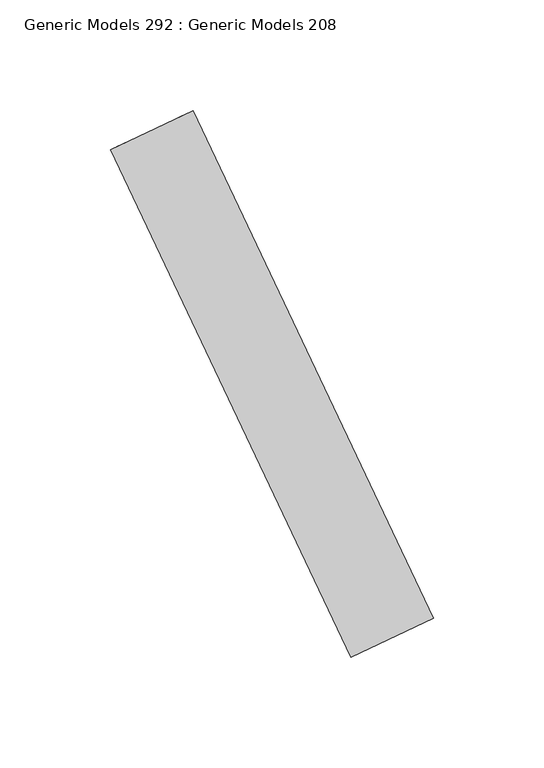
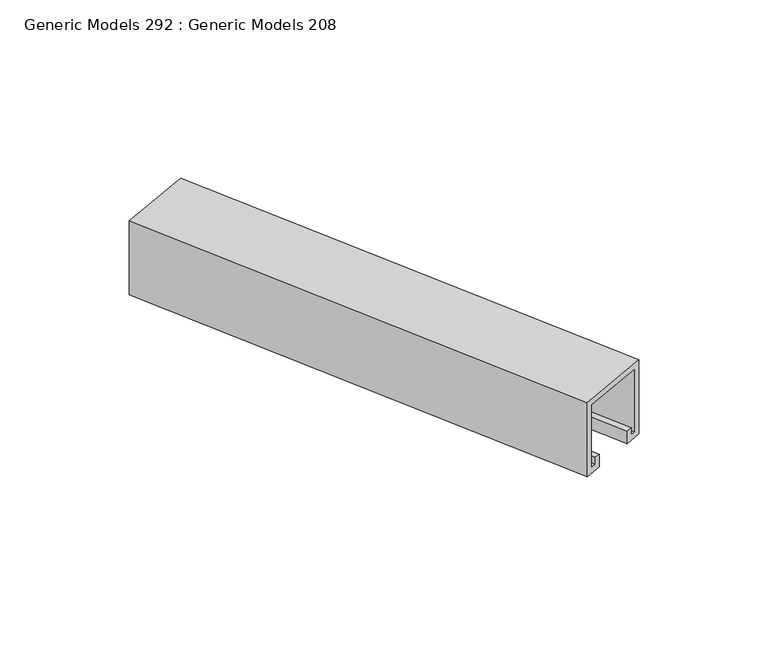
"""IFC4 building model written with IfcOpenShell, lengths in millimetres: proxy geometry, Generic Models 292 : Generic Models 208."""

from ifc_helpers import new_model, si_unit, frame, origin, place, context, project, spatial, polyline, outline, extrude, source, transform, mapped, element, save


def generic_models_292_generic_models_208_bf7aaf75(model_context):
    return source(origin(), model_context, "Body", "SweptSolid", [
        extrude(outline(polyline([(-3.175, 0.0), (-3.175, 34.925), (-38.1, 34.925), (-38.1, 31.75), (-34.13125, 31.75), (-34.13125, 28.575), (-41.275, 28.575), (-41.275, 38.1), (0.0, 38.1), (0.0, -3.175), (-41.275, -3.175), (-41.275, 6.35), (-34.13125, 6.35), (-34.13125, 3.175), (-38.1, 3.175), (-38.1, 0.0), (-3.175, 0.0)])), frame((-2064.1591152, -22579.8272705, 1035.05), z_axis=(-0.4281549299436163, 0.9037053479785195, 0.0), x_axis=(0.0, 0.0, 1.0)), (0.0, 0.0, 1.0), 254.0),
    ])


if __name__ == "__main__":
    model = new_model("IFC4")
    model_context = context("Model", 3, world=origin())
    ifc_project = project(units=[si_unit("LENGTHUNIT", "METRE", prefix="MILLI")], contexts=[model_context])
    site = spatial("IfcSite", under=ifc_project)
    building = spatial("IfcBuilding", under=site)
    placement = place(None, origin())
    generic_models_292_generic_models_208_shape = generic_models_292_generic_models_208_bf7aaf75(model_context)
    element("IfcBuildingElementProxy", 1, Name="Generic Models 292 : Generic Models 208", ObjectType="Generic Models 292 : Generic Models 208", at=placement, inside=building, context=model_context, shape_type="MappedRepresentation", body=[
        mapped(generic_models_292_generic_models_208_shape, transform((0.0, 0.0, 0.0), x_axis=(1.0, 0.0, 0.0), y_axis=(0.0, 1.0, 0.0), z_axis=(0.0, 0.0, 1.0))),
    ])
    save(model, "model.ifc")

# Revit data of these elements
# Element 1 (IfcBuildingElementProxy, "Generic Models 292 : Generic Models 208")
#   Materials on its faces: "UNISTRUT P1000, 1 5/8\" X 1 5/8\", CHANNEL OR ALUM. CHANNEL"
# Materials
#   "UNISTRUT P1000, 1 5/8\" X 1 5/8\", CHANNEL OR ALUM. CHANNEL": class "Metal", colour RGB 244 244 244, transparency 0, Description = "Aluminum 6061", Cost = 0
